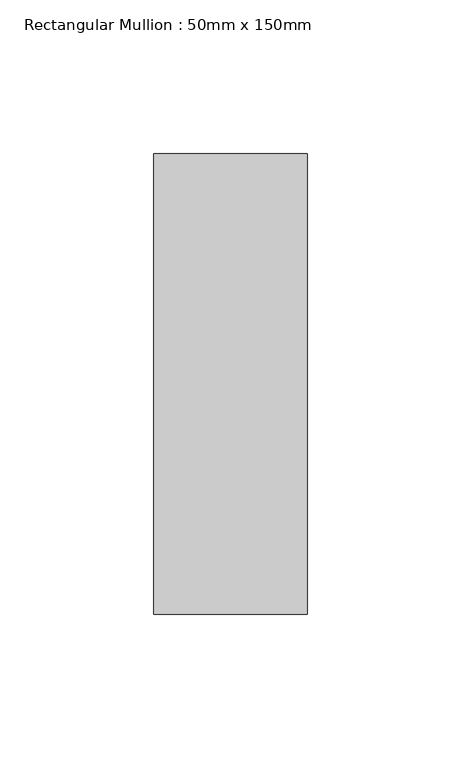
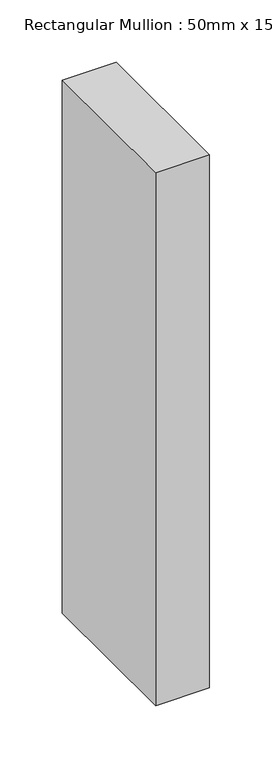
"""IFC4 building model written with IfcOpenShell, lengths in millimetres: member geometry, Rectangular Mullion : 50mm x 150mm."""

import ifcopenshell
import ifcopenshell.guid

model = None  # the IFC model being written
_history = None  # IfcOwnerHistory: only IFC2X3 demands one
_inside = {}  # id of a spatial element -> (the spatial element, [elements in it])
_under = {}  # id of a project, library or spatial element -> (it, [spatial elements below it])
_declared = {}  # id of a project -> (the project, [libraries it declares])
_typed = {}  # id of a type object -> (the type object, [elements of that type])
_made_of = {}  # id of a material, layer set ... -> (it, [elements and type objects made of it])


def new_model(schema):
    """Start an empty IFC model of exactly this schema.

    Asked for "IFC4X3", IfcOpenShell would pick the latest addendum, in which some entities
    have other attributes; the version numbers below select the first issue.
    IFC2X3 requires an IfcOwnerHistory on every rooted entity: one is made here for all.
    """
    global model, _history
    if schema == "IFC4X3":
        model = ifcopenshell.file(schema_version=(4, 3, 0, 0))
    else:
        model = ifcopenshell.file(schema=schema)
    _inside.clear()
    _under.clear()
    _declared.clear()
    _typed.clear()
    _made_of.clear()
    _history = None
    if model.schema == "IFC2X3":
        org = make("IfcOrganization", Name="unknown")
        user = make(
            "IfcPersonAndOrganization",
            ThePerson=make("IfcPerson", FamilyName="unknown"),
            TheOrganization=org,
        )
        app = make(
            "IfcApplication",
            ApplicationDeveloper=org,
            Version="unknown",
            ApplicationFullName="unknown",
            ApplicationIdentifier="unknown",
        )
        _history = make(
            "IfcOwnerHistory",
            OwningUser=user,
            OwningApplication=app,
            ChangeAction="ADDED",
            CreationDate=0,
        )
    return model


def make(cls, **values):
    """One entity of the class cls with the attributes given. An attribute that is None is left unset."""
    return model.create_entity(
        cls, **{name: value for name, value in values.items() if value is not None}
    )


def rooted(cls, **values):
    """An entity with a GlobalId (a new one), such as an element, a storey or a relation."""
    return make(cls, GlobalId=ifcopenshell.guid.new(), OwnerHistory=_history, **values)


def si_unit(unit_type, name, prefix=None):
    """IfcSIUnit, for example si_unit("LENGTHUNIT", "METRE", prefix="MILLI")."""
    return make("IfcSIUnit", UnitType=unit_type, Prefix=prefix, Name=name)


def assignment(units):
    """IfcUnitAssignment: the units of a project."""
    return None if units is None else make("IfcUnitAssignment", Units=units)


def point(xyz):
    """IfcCartesianPoint."""
    return None if xyz is None else make("IfcCartesianPoint", Coordinates=xyz)


def direction(xyz):
    """IfcDirection."""
    return None if xyz is None else make("IfcDirection", DirectionRatios=xyz)


def frame(location, z_axis=None, x_axis=None):
    """IfcAxis2Placement3D, a coordinate frame: its origin and axes. An axis left out is left unset."""
    return make(
        "IfcAxis2Placement3D",
        Location=point(location),
        Axis=direction(z_axis),
        RefDirection=direction(x_axis),
    )


def origin():
    """The frame at (0, 0, 0) with its axes left unset."""
    return frame((0.0, 0.0, 0.0))


def place(relative_to, where):
    """IfcLocalPlacement: puts the frame where relative to a parent placement (None: the world)."""
    return make(
        "IfcLocalPlacement", PlacementRelTo=relative_to, RelativePlacement=where
    )


def context(
    kind, dimensions, precision=None, world=None, true_north=None, identifier=None
):
    """IfcGeometricRepresentationContext, for example the 3D "Model" context."""
    return make(
        "IfcGeometricRepresentationContext",
        ContextIdentifier=identifier,
        ContextType=kind,
        CoordinateSpaceDimension=dimensions,
        Precision=precision,
        WorldCoordinateSystem=world,
        TrueNorth=true_north,
    )


def project(units=None, contexts=None):
    """IfcProject with its units and contexts."""
    return rooted(
        "IfcProject",
        Name="project",
        RepresentationContexts=contexts,
        UnitsInContext=assignment(units),
    )


def spatial(cls, under=None, at=None, **own):
    """A site, building, storey or space (cls), placed at a placement, below another one or the project."""
    s = rooted(cls, ObjectPlacement=at, **own)
    if under is not None:
        _under.setdefault(under.id(), (under, []))[1].append(s)
    return s


def polyline(points):
    """IfcPolyline through the points."""
    return make("IfcPolyline", Points=[point(p) for p in points])


def outline(outer, holes=None, kind="AREA"):
    """IfcArbitraryClosedProfileDef: a profile drawn as a closed curve; with holes, ...WithVoids."""
    if holes is None:
        return make("IfcArbitraryClosedProfileDef", ProfileType=kind, OuterCurve=outer)
    return make(
        "IfcArbitraryProfileDefWithVoids",
        ProfileType=kind,
        OuterCurve=outer,
        InnerCurves=holes,
    )


def extrude(swept, where, along, depth):
    """IfcExtrudedAreaSolid: the profile swept, set in the frame where, extruded along a direction by depth."""
    return make(
        "IfcExtrudedAreaSolid",
        SweptArea=swept,
        Position=where,
        ExtrudedDirection=direction(along),
        Depth=depth,
    )


def shape(context_of_items, identifier, shape_type, items):
    """IfcShapeRepresentation: the items that make up one representation, for example the "Body"."""
    return make(
        "IfcShapeRepresentation",
        ContextOfItems=context_of_items,
        RepresentationIdentifier=identifier,
        RepresentationType=shape_type,
        Items=items,
    )


def source(mapping_origin, context_of_items, identifier, shape_type, items):
    """IfcRepresentationMap: a shape defined once, which mapped items show again and again."""
    return make(
        "IfcRepresentationMap",
        MappingOrigin=mapping_origin,
        MappedRepresentation=shape(context_of_items, identifier, shape_type, items),
    )


def transform(
    local_origin,
    x_axis=None,
    y_axis=None,
    z_axis=None,
    scale=None,
    scale2=None,
    scale3=None,
    uniform=True,
):
    """IfcCartesianTransformationOperator3D, or its non-uniform kind. x_axis, y_axis, z_axis: its Axis1, 2, 3."""
    if uniform:
        return make(
            "IfcCartesianTransformationOperator3D",
            Axis1=direction(x_axis),
            Axis2=direction(y_axis),
            LocalOrigin=point(local_origin),
            Scale=scale,
            Axis3=direction(z_axis),
        )
    return make(
        "IfcCartesianTransformationOperator3DnonUniform",
        Axis1=direction(x_axis),
        Axis2=direction(y_axis),
        LocalOrigin=point(local_origin),
        Scale=scale,
        Axis3=direction(z_axis),
        Scale2=scale2,
        Scale3=scale3,
    )


def mapped(mapping_source, mapping_target):
    """IfcMappedItem: shows the shape of a source again, moved by a transform."""
    return make(
        "IfcMappedItem", MappingSource=mapping_source, MappingTarget=mapping_target
    )


def made_of(thing, what):
    """Note that an element or type object is made of a material, layer set ...; save() writes the relation."""
    if what is not None:
        _made_of.setdefault(what.id(), (what, []))[1].append(thing)
    return thing


def element(
    cls,
    number,
    at=None,
    inside=None,
    cuts=None,
    type_object=None,
    material=None,
    context=None,
    identifier="Body",
    shape_type=None,
    held_by="IfcProductDefinitionShape",
    body=None,
    shapes=None,
    **own,
):
    """One element of the class cls, such as IfcWall. Its Tag is "e" and its number.

    at: its placement. inside: the storey or other place that contains it. cuts: it is an
    opening in that element (IfcRelVoidsElement). A single representation is given by context,
    identifier, shape_type and body (its items); several are given by shapes. held_by: the class
    of the entity that holds the representations. save() writes the other relations.
    """
    e = rooted(cls, Tag="e%d" % number, ObjectPlacement=at, **own)
    if body is not None:
        shapes = [shape(context, identifier, shape_type, body)]
    if shapes is not None:
        e.Representation = make(held_by, Representations=shapes)
    if inside is not None:
        _inside.setdefault(inside.id(), (inside, []))[1].append(e)
    if cuts is not None:
        rooted(
            "IfcRelVoidsElement", RelatingBuildingElement=cuts, RelatedOpeningElement=e
        )
    if type_object is not None:
        _typed.setdefault(type_object.id(), (type_object, []))[1].append(e)
    return made_of(e, material)


def aggregate(whole, parts):
    """IfcRelAggregates: a whole, such as a stair, and the parts it consists of."""
    return rooted("IfcRelAggregates", RelatingObject=whole, RelatedObjects=parts)


def save(model, path):
    """Write the relations noted so far, then the file.

    IfcRelAggregates (storeys below a building ...), IfcRelContainedInSpatialStructure (elements
    in a storey), IfcRelDefinesByType, IfcRelAssociatesMaterial and IfcRelDeclares: one each for
    every whole, place, type object, material and project.
    """
    for whole, parts in _under.values():
        aggregate(whole, parts)
    for where, things in _inside.values():
        rooted(
            "IfcRelContainedInSpatialStructure",
            RelatedElements=things,
            RelatingStructure=where,
        )
    for kind, things in _typed.values():
        rooted("IfcRelDefinesByType", RelatedObjects=things, RelatingType=kind)
    for what, things in _made_of.values():
        rooted("IfcRelAssociatesMaterial", RelatedObjects=things, RelatingMaterial=what)
    for by, libraries in _declared.values():
        rooted("IfcRelDeclares", RelatingContext=by, RelatedDefinitions=libraries)
    model.write(path)


def rectangular_mullion_50mm_x_150mm_e851a0b8(model_context):
    return source(origin(), model_context, "Body", "SweptSolid", [
        extrude(outline(polyline([(0.0, 75.0), (0.0, -75.0), (-50.0, -75.0), (-50.0, 75.0), (0.0, 75.0)])), frame((0.0, 0.0, -522.7272727), z_axis=(0.0, 0.0, 1.0), x_axis=(1.0, 0.0, 0.0)), (0.0, 0.0, 1.0), 522.7272727),
    ])


if __name__ == "__main__":
    model = new_model("IFC4")
    model_context = context("Model", 3, world=origin())
    ifc_project = project(units=[si_unit("LENGTHUNIT", "METRE", prefix="MILLI")], contexts=[model_context])
    site = spatial("IfcSite", under=ifc_project)
    building = spatial("IfcBuilding", under=site)
    placement = place(None, origin())
    rectangular_mullion_50mm_x_150mm_shape = rectangular_mullion_50mm_x_150mm_e851a0b8(model_context)
    element("IfcMember", 1, ObjectType="Rectangular Mullion : 50mm x 150mm", at=placement, inside=building, context=model_context, shape_type="MappedRepresentation", body=[
        mapped(rectangular_mullion_50mm_x_150mm_shape, transform((0.0, 0.0, 0.0), x_axis=(1.0, 0.0, 0.0), y_axis=(0.0, 1.0, 0.0), z_axis=(0.0, 0.0, 1.0))),
    ])
    save(model, "model.ifc")

# Revit data of these elements
# Type "Rectangular Mullion : 50mm x 150mm"
#   built-in parameter 1007304 = 0.492126 (stored number, unit not read)
#   built-in parameter 1007301 = 0.082021 (stored number, unit not read)
#   built-in parameter 1007300 = 0.082021 (stored number, unit not read)
# Element 1 (IfcMember, "Rectangular Mullion : 50mm x 150mm")
#   Materials on its faces: "Aluminum"
# Materials
#   "Aluminum": class "Metal", colour RGB 244 244 244, transparency 0, Description = "Aluminum 6061", Cost = 0
